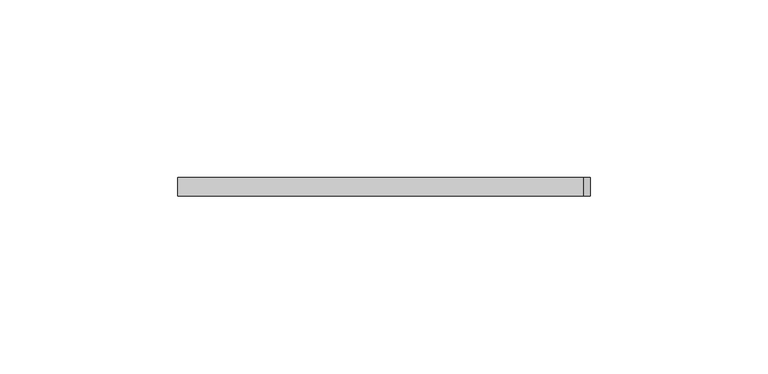
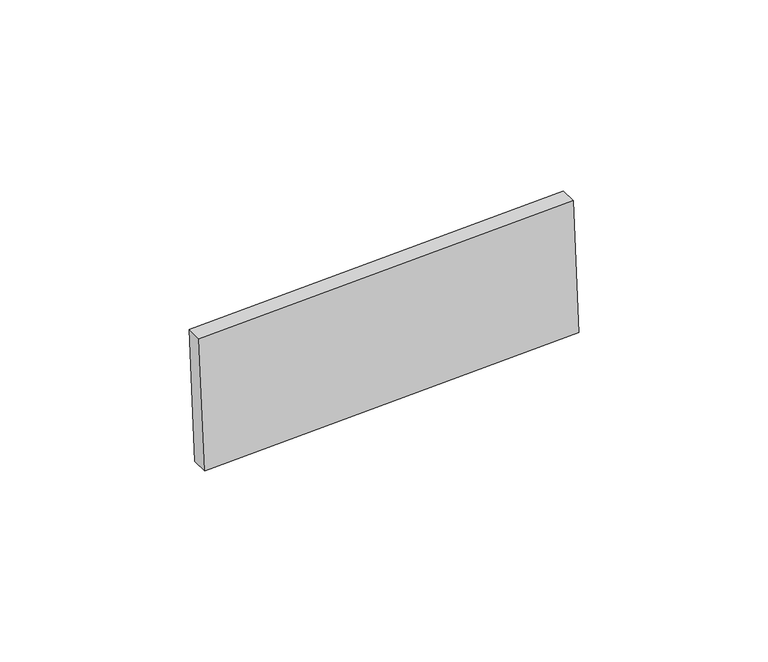
"""IFC4 building model written with IfcOpenShell, lengths in millimetres: proxy geometry, Inner panel:Inner panel:1:Inner panel:1 : Inner panel:Inner panel:300324:2:Inner panel:1:Inner panel:1 : Inner panel:Inner panel:300324:2 : Inner panel:Inner panel:1:Inner panel:1 : Inner panel:Inner panel:300324:300043:169 : Inner panel:Inner panel:1:Inner panel:1 : Inner panel:Inner panel:300324:2:Inner panel:1:Inner panel:1 : Inner panel:Inner panel:300324:2 : Inner panel:Inner panel:1:Inner panel:1 : Inner panel:Inner panel:300324:300043:308120."""

from ifc_helpers import new_model, si_unit, frame, origin, place, context, project, spatial, polyline, outline, extrude, source, transform, mapped, element, save


def generic_models_6f7d9f27(model_context):
    return source(origin(), model_context, "Body", "SweptSolid", [
        extrude(outline(polyline([(0.0, -114.3), (0.0, 0.0), (5.213809, 0.0), (5.213809, -114.3), (0.0, -114.3)])), frame((560425.2415304, -566213.307991, 3954.8593665), z_axis=(-0.04163054471216399, 0.0, 0.9991330730923527), x_axis=(0.0, -1.0, 0.0)), (0.0, 0.0, 1.0), 43.2233908),
    ])


if __name__ == "__main__":
    model = new_model("IFC4")
    model_context = context("Model", 3, world=origin())
    ifc_project = project(units=[si_unit("LENGTHUNIT", "METRE", prefix="MILLI")], contexts=[model_context])
    site = spatial("IfcSite", under=ifc_project)
    building = spatial("IfcBuilding", under=site)
    placement = place(None, origin())
    generic_models_shape = generic_models_6f7d9f27(model_context)
    element("IfcBuildingElementProxy", 1, Name="Inner panel:Inner panel:1:Inner panel:1 : Inner panel:Inner panel:300324:2:Inner panel:1:Inner panel:1 : Inner panel:Inner panel:300324:2 : Inner panel:Inner panel:1:Inner panel:1 : Inner panel:Inner panel:300324:300043:169 : Inner panel:Inner panel:1:Inner panel:1 : Inner panel:Inner panel:300324:2:Inner panel:1:Inner panel:1 : Inner panel:Inner panel:300324:2 : Inner panel:Inner panel:1:Inner panel:1 : Inner panel:Inner panel:300324:300043:308120", ObjectType="Inner panel:Inner panel:1:Inner panel:1 : Inner panel:Inner panel:300324:2:Inner panel:1:Inner panel:1 : Inner panel:Inner panel:300324:2 : Inner panel:Inner panel:1:Inner panel:1 : Inner panel:Inner panel:300324:300043:169 : Inner panel:Inner panel:1:Inner panel:1 : Inner panel:Inner panel:300324:2:Inner panel:1:Inner panel:1 : Inner panel:Inner panel:300324:2 : Inner panel:Inner panel:1:Inner panel:1 : Inner panel:Inner panel:300324:300043:308120", at=placement, inside=building, context=model_context, shape_type="MappedRepresentation", body=[
        mapped(generic_models_shape, transform((0.0, 0.0, 0.0), x_axis=(1.0, 0.0, 0.0), y_axis=(0.0, 1.0, 0.0), z_axis=(0.0, 0.0, 1.0))),
    ])
    save(model, "model.ifc")

# Revit data of these elements
# Type "Inner panel:Inner panel:1:Inner panel:1 : Inner panel:Inner panel:300324:2:Inner panel:1:Inner panel:1 : Inner panel:Inner panel:300324:2 : Inner panel:Inner panel:1:Inner panel:1 : Inner panel:Inner panel:300324:300043:169 : Inner panel:Inner panel:1:Inner panel:1 : Inner panel:Inner panel:300324:2:Inner panel:1:Inner panel:1 : Inner panel:Inner panel:300324:2 : Inner panel:Inner panel:1:Inner panel:1 : Inner panel:Inner panel:300324:300043:308120"
#   NameOverride = "Inner panel:Inner panel:1:Inner panel:1 : Inner panel:Inner panel:300324:2:Inner panel:1:Inner panel:1 : Inner panel:Inner panel:300324:2 : Inner panel:Inner panel:1:Inner panel:1 : Inner panel:Inner panel:300324:300043:308120"
#   ObjectTypeOverride = "Inner panel:1:Inner panel:1 : Inner panel:Inner panel:300324:2 : Inner panel:Inner panel:1:Inner panel:1 : Inner panel:Inner panel:300324:300043"
#   Reference = "Inner panel"
#   Tag = "308120"
# Element 1 (IfcBuildingElementProxy, "Inner panel:Inner panel:1:Inner panel:1 : Inner panel:Inner panel:300324:2:Inner panel:1:Inner panel:1 : Inner panel:Inner panel:300324:2 : Inner panel:Inner panel:1:Inner panel:1 : Inner panel:Inner panel:300324:300043:169 : Inner panel:Inner panel:1:Inner panel:1 : Inner panel:Inner panel:300324:2:Inner panel:1:Inner panel:1 : Inner panel:Inner panel:300324:2 : Inner panel:Inner panel:1:Inner panel:1 : Inner panel:Inner panel:300324:300043:308120")
#   Materials on its faces: "SLIDING CLIP"
# Materials
#   "SLIDING CLIP": class "Generic", colour RGB 120 120 120, transparency 0, Cost = 0
